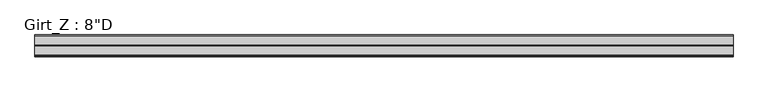
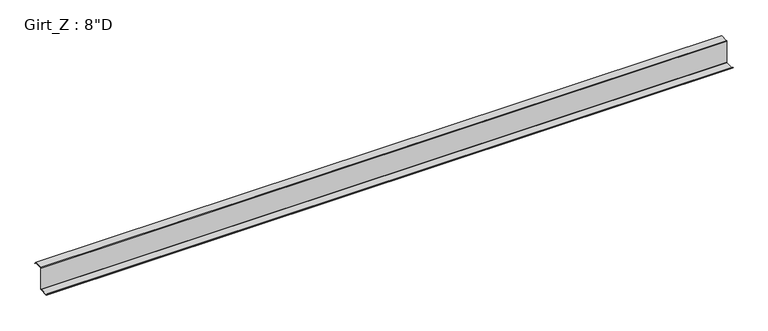
"""IFC4 building model written with IfcOpenShell, lengths in millimetres: beam geometry."""

from ifc_helpers import new_model, si_unit, point, frame, frame_2d, origin, place, context, project, spatial, polyline, circle_curve, trimmed, segment, composite_curve, outline, extrude, source, transform, mapped, element, save


def beam_fb9fe81b(model_context):
    return source(origin(), model_context, "Body", "SweptSolid", [
        extrude(outline(composite_curve([segment(polyline([(77.9859375, 101.6), (90.2310415, 87.0068534), (88.1028742, 85.221109), (76.6904765, 98.821875), (3.3005807, 98.821875)]), True, "CONTINUOUS"), segment(trimmed(circle_curve(frame_2d((3.3741066, 96.8381931)), 1.9850441), [point((3.3005807, 98.821875))], [point((1.3890625, 96.8381931))], True, "CARTESIAN"), True, "CONTINUOUS"), segment(polyline([(1.3890625, 96.8381931), (1.3890625, -101.6), (-84.3359375, -101.6), (-96.5810415, -87.0068534), (-94.4528742, -85.221109), (-83.0404765, -98.821875), (-3.2694106, -98.821875)]), True, "CONTINUOUS"), segment(trimmed(circle_curve(frame_2d((-3.3748024, -96.8389339)), 1.9857399), [point((-3.2694106, -98.821875))], [point((-1.3890625, -96.8389339))], True, "CARTESIAN"), True, "CONTINUOUS"), segment(polyline([(-1.3890625, -96.8389339), (-1.3890625, 96.8375)]), True, "CONTINUOUS"), segment(trimmed(circle_curve(frame_2d((3.3734375, 96.8375)), 4.7625), [point((-1.3890625, 96.8375))], [point((3.3734375, 101.6))], False, "CARTESIAN"), True, "CONTINUOUS"), segment(polyline([(3.3734375, 101.6), (77.9859375, 101.6)]), True, "CONTINUOUS")], self_intersect=False)), frame((-2884.4875, 0.0, 0.0), z_axis=(1.0, 0.0, 0.0), x_axis=(0.0, 1.0, 0.0)), (0.0, 0.0, 1.0), 5984.875),
    ])


if __name__ == "__main__":
    model = new_model("IFC4")
    model_context = context("Model", 3, world=origin())
    ifc_project = project(units=[si_unit("LENGTHUNIT", "METRE", prefix="MILLI")], contexts=[model_context])
    site = spatial("IfcSite", under=ifc_project)
    building = spatial("IfcBuilding", under=site)
    placement = place(None, origin())
    beam_shape = beam_fb9fe81b(model_context)
    element("IfcBeam", 1, ObjectType="Girt_Z : 8\"D", at=placement, inside=building, context=model_context, shape_type="MappedRepresentation", body=[
        mapped(beam_shape, transform((0.0, 0.0, 0.0), x_axis=(1.0, 0.0, 0.0), y_axis=(0.0, 1.0, 0.0), z_axis=(0.0, 0.0, 1.0))),
    ])
    save(model, "model.ifc")

# Revit data of these elements
# Type "Girt_Z : 8\"D"
#   half leg = 0' - 1 11/16"
#   Web_Thickness = 0' - 0 7/64"
#   Length [instance default] = 10' - 0"
#   Leg_2 = 0' - 3 3/8"
#   Leg_1 = 0' - 3 1/8"
#   Height = 0' - 8"
#   Structural Material [instance default] = none
